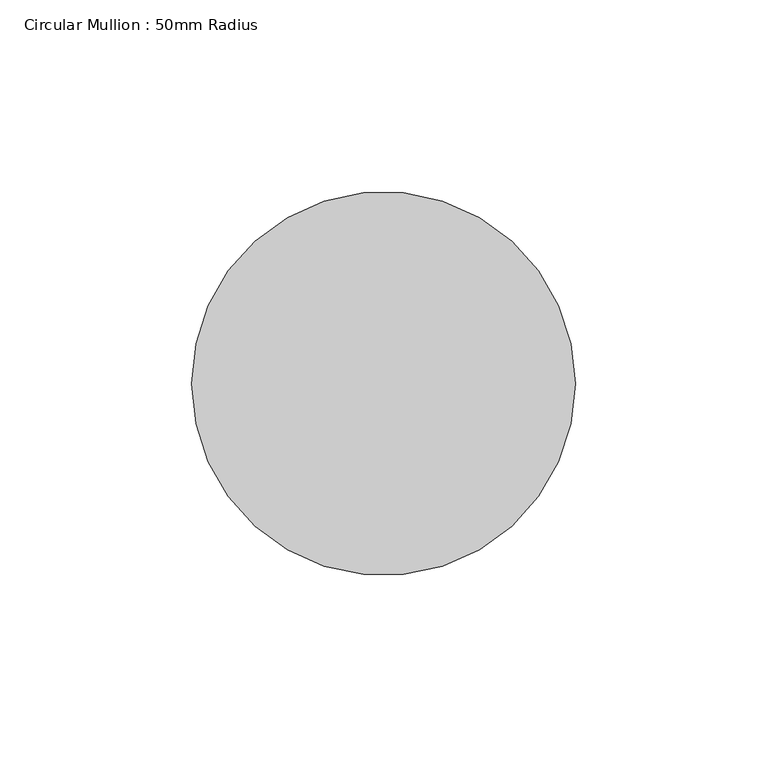
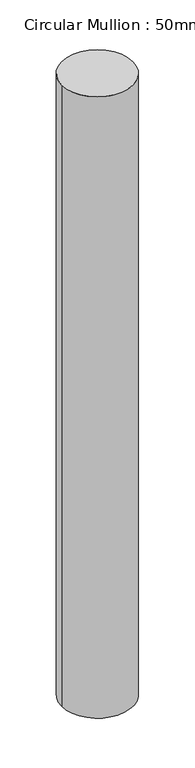
"""IFC4 building model written with IfcOpenShell, lengths in millimetres: member geometry, Circular Mullion : 50mm Radius."""

from ifc_helpers import new_model, si_unit, point, frame, origin, origin_2d, place, context, project, spatial, circle_curve, trimmed, segment, composite_curve, outline, extrude, source, transform, mapped, element, save


def circular_mullion_50mm_radius_9e6aeb12(model_context):
    return source(origin(), model_context, "Body", "SweptSolid", [
        extrude(outline(composite_curve([segment(trimmed(circle_curve(origin_2d(), 50.0), [point((50.0, 0.0))], [point((-50.0, 0.0))], False, "CARTESIAN"), True, "CONTINUOUS"), segment(trimmed(circle_curve(origin_2d(), 50.0), [point((-50.0, 0.0))], [point((50.0, 0.0))], False, "CARTESIAN"), True, "CONTINUOUS")], self_intersect=False)), frame((0.0, 0.0, -921.7882586), z_axis=(0.0, 0.0, 1.0), x_axis=(1.0, 0.0, 0.0)), (0.0, 0.0, 1.0), 921.7882586),
    ])


if __name__ == "__main__":
    model = new_model("IFC4")
    model_context = context("Model", 3, world=origin())
    ifc_project = project(units=[si_unit("LENGTHUNIT", "METRE", prefix="MILLI")], contexts=[model_context])
    site = spatial("IfcSite", under=ifc_project)
    building = spatial("IfcBuilding", under=site)
    placement = place(None, origin())
    circular_mullion_50mm_radius_shape = circular_mullion_50mm_radius_9e6aeb12(model_context)
    element("IfcMember", 1, ObjectType="Circular Mullion : 50mm Radius", at=placement, inside=building, context=model_context, shape_type="MappedRepresentation", body=[
        mapped(circular_mullion_50mm_radius_shape, transform((0.0, 0.0, 0.0), x_axis=(1.0, 0.0, 0.0), y_axis=(0.0, 1.0, 0.0), z_axis=(0.0, 0.0, 1.0))),
    ])
    save(model, "model.ifc")

# Revit data of these elements
# Type "Circular Mullion : 50mm Radius"
#   built-in parameter 1007350 = 0.164042 (stored number, unit not read)
# Element 1 (IfcMember, "Circular Mullion : 50mm Radius")
#   Materials on its faces: "Aluminium"
# Materials
#   "Aluminium": class "Metal", colour RGB 247 247 247, transparency 0, Description = "Aluminium 6061", Cost = 0
